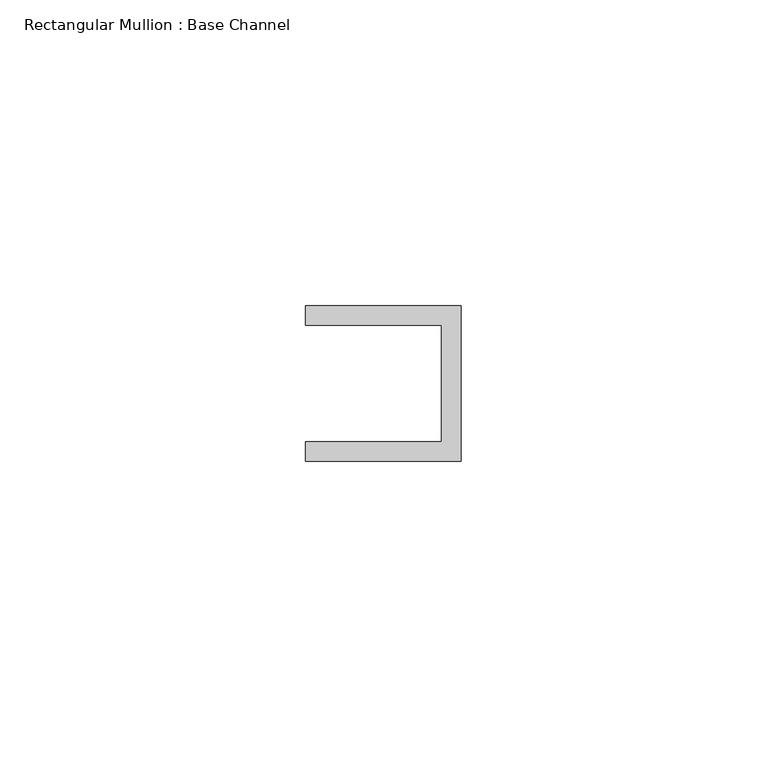
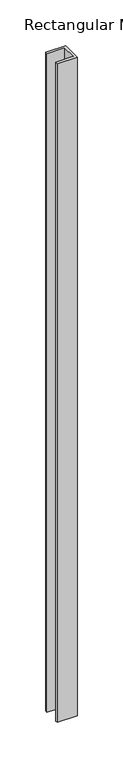
"""IFC4 building model written with IfcOpenShell, lengths in millimetres: member geometry, Rectangular Mullion : Base Channel."""

from ifc_helpers import new_model, si_unit, frame, origin, place, context, project, spatial, polyline, outline, extrude, source, transform, mapped, element, save


def rectangular_mullion_base_channel_0040bc96(model_context):
    return source(origin(), model_context, "Body", "SweptSolid", [
        extrude(outline(polyline([(0.0, -12.7), (-25.4, -12.7), (-25.4, -9.525), (-3.175, -9.525), (-3.175, 9.525), (-25.4, 9.525), (-25.4, 12.7), (0.0, 12.7), (0.0, -12.7)])), frame((0.0, 0.0, -883.3407348), z_axis=(0.0, 0.0, 1.0), x_axis=(1.0, 0.0, 0.0)), (0.0, 0.0, 1.0), 883.3407348),
    ])


if __name__ == "__main__":
    model = new_model("IFC4")
    model_context = context("Model", 3, world=origin())
    ifc_project = project(units=[si_unit("LENGTHUNIT", "METRE", prefix="MILLI")], contexts=[model_context])
    site = spatial("IfcSite", under=ifc_project)
    building = spatial("IfcBuilding", under=site)
    placement = place(None, origin())
    rectangular_mullion_base_channel_shape = rectangular_mullion_base_channel_0040bc96(model_context)
    element("IfcMember", 1, ObjectType="Rectangular Mullion : Base Channel", at=placement, inside=building, context=model_context, shape_type="MappedRepresentation", body=[
        mapped(rectangular_mullion_base_channel_shape, transform((0.0, 0.0, 0.0), x_axis=(1.0, 0.0, 0.0), y_axis=(0.0, 1.0, 0.0), z_axis=(0.0, 0.0, 1.0))),
    ])
    save(model, "model.ifc")

# Revit data of these elements
# Type "Rectangular Mullion : Base Channel"
#   built-in parameter 1007322 = 0.0833333 (stored number, unit not read)
#   built-in parameter 1007321 = 0.0416667 (stored number, unit not read)
#   built-in parameter 1007320 = -0.03125 (stored number, unit not read)
# Element 1 (IfcMember, "Rectangular Mullion : Base Channel")
#   Materials on its faces: "ALUM"
# Materials
#   "ALUM": class "Generic", colour RGB 157 157 157, transparency 0, Cost = 0
